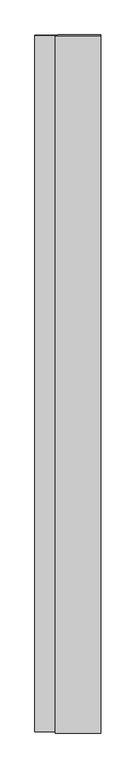
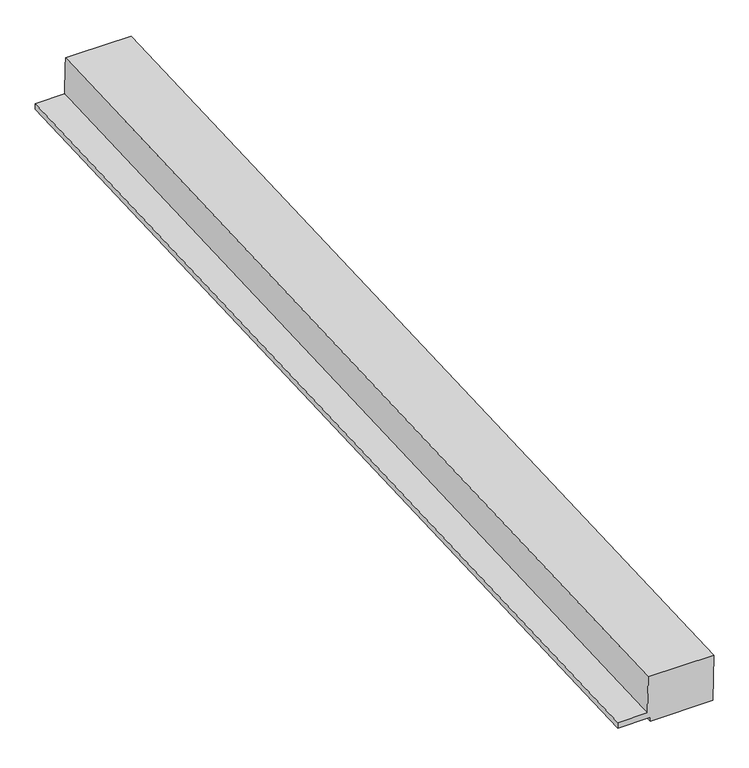
"""IFC4 building model written with IfcOpenShell, lengths in millimetres: proxy geometry, Generic Models 7:Generic Models 1:1:Generic Models 1:1 : Generic Models 7:Generic Models 1:337419:55 : Generic Models 7:Generic Models 1:1:Generic Models 1:1 : Generic Models 7:Generic Models 1:337419:306201."""

from ifc_helpers import new_model, si_unit, origin, place, context, project, spatial, faceted_brep, source, transform, mapped, element, save


def generic_models_9d84b857(model_context):
    return source(origin(), model_context, "Body", "Brep", [
        faceted_brep([(579263.458906, -573934.7533936, 3881.3366715), (579263.458906, -573935.6047024, 3901.7680827), (579104.5117239, -573935.6047024, 3901.7680827), (579104.5117239, -573936.8004003, 3930.4648304), (579247.1208806, -573936.8004003, 3930.4648304), (579247.1208806, -573942.9163841, 4077.2484422), (579247.1208806, -573944.6255932, 4118.2694601), (579304.933599, -573944.6255932, 4118.2694601), (579564.6208806, -573944.6255932, 4118.2694601), (579564.6208806, -573934.7533936, 3881.3366715), (579263.458906, -578807.3255645, 3678.312831), (579564.6208806, -578807.3255645, 3678.312831), (579564.6208806, -578817.197764, 3915.2456196), (579247.1208806, -578817.197764, 3915.2456196), (579247.1208806, -578809.3725711, 3727.44099), (579104.5117239, -578809.3725711, 3727.44099), (579104.5117239, -578808.1768733, 3698.7442422), (579263.458906, -578808.1768733, 3698.7442422), (579247.1208806, -577227.6325678, 3981.4775028)], [[[0, 1, 2, 3, 4, 5, 6, 7, 8, 9]], [[10, 11, 12, 13, 14, 15, 16, 17]], [[1, 0, 10, 17]], [[2, 1, 17, 16]], [[3, 2, 16, 15]], [[4, 3, 15, 14]], [[6, 5, 4, 14, 13, 18]], [[8, 7, 6, 18, 13, 12]], [[9, 8, 12, 11]], [[0, 9, 11, 10]]]),
    ])


if __name__ == "__main__":
    model = new_model("IFC4")
    model_context = context("Model", 3, world=origin())
    ifc_project = project(units=[si_unit("LENGTHUNIT", "METRE", prefix="MILLI")], contexts=[model_context])
    site = spatial("IfcSite", under=ifc_project)
    building = spatial("IfcBuilding", under=site)
    placement = place(None, origin())
    generic_models_shape = generic_models_9d84b857(model_context)
    element("IfcBuildingElementProxy", 1, Name="Generic Models 7:Generic Models 1:1:Generic Models 1:1 : Generic Models 7:Generic Models 1:337419:55 : Generic Models 7:Generic Models 1:1:Generic Models 1:1 : Generic Models 7:Generic Models 1:337419:306201", ObjectType="Generic Models 7:Generic Models 1:1:Generic Models 1:1 : Generic Models 7:Generic Models 1:337419:55 : Generic Models 7:Generic Models 1:1:Generic Models 1:1 : Generic Models 7:Generic Models 1:337419:306201", at=placement, inside=building, context=model_context, shape_type="MappedRepresentation", body=[
        mapped(generic_models_shape, transform((0.0, 0.0, 0.0), x_axis=(1.0, 0.0, 0.0), y_axis=(0.0, 1.0, 0.0), z_axis=(0.0, 0.0, 1.0))),
    ])
    save(model, "model.ifc")

# Revit data of these elements
# Type "Generic Models 7:Generic Models 1:1:Generic Models 1:1 : Generic Models 7:Generic Models 1:337419:55 : Generic Models 7:Generic Models 1:1:Generic Models 1:1 : Generic Models 7:Generic Models 1:337419:306201"
#   NameOverride = "Generic Models 7:Generic Models 1:1:Generic Models 1:1 : Generic Models 7:Generic Models 1:337419:306201"
#   ObjectTypeOverride = "Generic Models 1:1 : Generic Models 7:Generic Models 1:337419"
#   Reference = "Generic Models 1"
#   Tag = "306201"
# Element 1 (IfcBuildingElementProxy, "Generic Models 7:Generic Models 1:1:Generic Models 1:1 : Generic Models 7:Generic Models 1:337419:55 : Generic Models 7:Generic Models 1:1:Generic Models 1:1 : Generic Models 7:Generic Models 1:337419:306201")
#   Materials on its faces: "FULL CAVITY CLASS A FIBERGLASS INSULATION WITH DURABLE VAPOR BARRIER (BLACK) LINER"
# Materials
#   "FULL CAVITY CLASS A FIBERGLASS INSULATION WITH DURABLE VAPOR BARRIER (BLACK) LINER": class "Unassigned", colour RGB 158 92 175, transparency 0, Cost = 0
